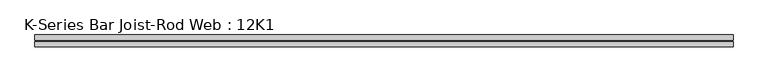
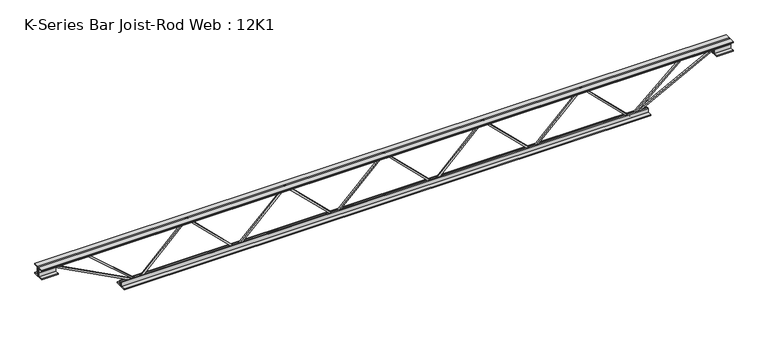
"""IFC4 building model written with IfcOpenShell, lengths in millimetres: beam geometry, K-Series Bar Joist-Rod Web : 12K1."""

from ifc_helpers import new_model, si_unit, frame, origin, place, context, project, spatial, polyline, outline, extrude, source, transform, mapped, element, save


def k_series_bar_joist_rod_web_12k1_62c0aeb9(model_context):
    return source(origin(), model_context, "Body", "SweptSolid", [
        extrude(outline(polyline([(-141.2875, 304.00625), (-150.8125, 304.00625), (-150.8125, 309.1277103), (141.2875, 606.7839603), (141.2875, 609.2410397), (-150.8125, 906.8972897), (-150.8125, 912.01875), (-141.2875, 912.01875), (-141.2875, 910.7902103), (150.8125, 613.1339603), (150.8125, 602.8910397), (-141.2875, 305.2347897), (-141.2875, 304.00625)])), frame((0.0, -4.7625, 0.0), z_axis=(0.0, 1.0, 0.0), x_axis=(0.0, 0.0, 1.0)), (0.0, 0.0, 1.0), 9.525),
        extrude(outline(polyline([(-141.2875, -304.00625), (-150.8125, -304.00625), (-150.8125, -298.8847897), (141.2875, -1.2285397), (141.2875, 1.2285397), (-150.8125, 298.8847897), (-150.8125, 304.00625), (-141.2875, 304.00625), (-141.2875, 302.7777103), (150.8125, 5.1214603), (150.8125, -5.1214603), (-141.2875, -302.7777103), (-141.2875, -304.00625)])), frame((0.0, -4.7625, 0.0), z_axis=(0.0, 1.0, 0.0), x_axis=(0.0, 0.0, 1.0)), (0.0, 0.0, 1.0), 9.525),
        extrude(outline(polyline([(-141.2875, -912.01875), (-150.8125, -912.01875), (-150.8125, -906.8972897), (141.2875, -609.2410397), (141.2875, -606.7839603), (-150.8125, -309.1277103), (-150.8125, -304.00625), (-141.2875, -304.00625), (-141.2875, -305.2347897), (150.8125, -602.8910397), (150.8125, -613.1339603), (-141.2875, -910.7902103), (-141.2875, -912.01875)])), frame((0.0, -4.7625, 0.0), z_axis=(0.0, 1.0, 0.0), x_axis=(0.0, 0.0, 1.0)), (0.0, 0.0, 1.0), 9.525),
        extrude(outline(polyline([(-141.2875, 912.01875), (-150.8125, 912.01875), (-150.8125, 917.1402103), (141.2875, 1214.7964603), (141.2875, 1217.2535397), (-150.8125, 1514.9097897), (-150.8125, 1520.03125), (-141.2875, 1520.03125), (-141.2875, 1518.8027103), (150.8125, 1221.1464603), (150.8125, 1210.9035397), (-141.2875, 913.2472897), (-141.2875, 912.01875)])), frame((0.0, -4.7625, 0.0), z_axis=(0.0, 1.0, 0.0), x_axis=(0.0, 0.0, 1.0)), (0.0, 0.0, 1.0), 9.525),
        extrude(outline(polyline([(-141.2875, -1520.03125), (-150.8125, -1520.03125), (-150.8125, -1514.9097897), (141.2875, -1217.2535397), (141.2875, -1214.7964603), (-150.8125, -917.1402103), (-150.8125, -912.01875), (-141.2875, -912.01875), (-141.2875, -913.2472897), (150.8125, -1210.9035397), (150.8125, -1221.1464603), (-141.2875, -1518.8027103), (-141.2875, -1520.03125)])), frame((0.0, -4.7625, 0.0), z_axis=(0.0, 1.0, 0.0), x_axis=(0.0, 0.0, 1.0)), (0.0, 0.0, 1.0), 9.525),
        extrude(outline(polyline([(4.7625, 152.4), (36.5125, 152.4), (36.5125, 146.05), (11.1125, 146.05), (11.1125, 120.65), (4.7625, 120.65), (4.7625, 152.4)])), frame((-2129.63125, 0.0, 0.0), z_axis=(1.0, 0.0, 0.0), x_axis=(0.0, 1.0, 0.0)), (0.0, 0.0, 1.0), 4259.2625),
        extrude(outline(polyline([(-4.7625, 152.4), (-4.7625, 120.65), (-11.1125, 120.65), (-11.1125, 146.05), (-36.5125, 146.05), (-36.5125, 152.4), (-4.7625, 152.4)])), frame((-2129.63125, 0.0, 0.0), z_axis=(1.0, 0.0, 0.0), x_axis=(0.0, 1.0, 0.0)), (0.0, 0.0, 1.0), 4259.2625),
        extrude(outline(polyline([(-4.7625, 88.9), (-36.5125, 88.9), (-36.5125, 95.25), (-11.1125, 95.25), (-11.1125, 120.65), (-4.7625, 120.65), (-4.7625, 88.9)])), frame((-2129.63125, 0.0, 0.0), z_axis=(1.0, 0.0, 0.0), x_axis=(0.0, 1.0, 0.0)), (0.0, 0.0, 1.0), 101.6),
        extrude(outline(polyline([(36.5125, 88.9), (4.7625, 88.9), (4.7625, 120.65), (11.1125, 120.65), (11.1125, 95.25), (36.5125, 95.25), (36.5125, 88.9)])), frame((-2129.63125, 0.0, 0.0), z_axis=(1.0, 0.0, 0.0), x_axis=(0.0, 1.0, 0.0)), (0.0, 0.0, 1.0), 101.6),
        extrude(outline(polyline([(4.7625, 88.9), (4.7625, 120.65), (11.1125, 120.65), (11.1125, 95.25), (36.5125, 95.25), (36.5125, 88.9), (4.7625, 88.9)])), frame((2028.03125, 0.0, 0.0), z_axis=(1.0, 0.0, 0.0), x_axis=(0.0, 1.0, 0.0)), (0.0, 0.0, 1.0), 101.6),
        extrude(outline(polyline([(-4.7625, 88.9), (-36.5125, 88.9), (-36.5125, 95.25), (-11.1125, 95.25), (-11.1125, 120.65), (-4.7625, 120.65), (-4.7625, 88.9)])), frame((2028.03125, 0.0, 0.0), z_axis=(1.0, 0.0, 0.0), x_axis=(0.0, 1.0, 0.0)), (0.0, 0.0, 1.0), 101.6),
        extrude(outline(polyline([(4.7625, -152.4), (4.7625, -120.65), (11.1125, -120.65), (11.1125, -146.05), (36.5125, -146.05), (36.5125, -152.4), (4.7625, -152.4)])), frame((-1621.63125, 0.0, 0.0), z_axis=(1.0, 0.0, 0.0), x_axis=(0.0, 1.0, 0.0)), (0.0, 0.0, 1.0), 3243.2625),
        extrude(outline(polyline([(-4.7625, -152.4), (-36.5125, -152.4), (-36.5125, -146.05), (-11.1125, -146.05), (-11.1125, -120.65), (-4.7625, -120.65), (-4.7625, -152.4)])), frame((-1621.63125, 0.0, 0.0), z_axis=(1.0, 0.0, 0.0), x_axis=(0.0, 1.0, 0.0)), (0.0, 0.0, 1.0), 3243.2625),
        extrude(outline(polyline([(0.0, -9.525), (0.0, 0.0), (573.7533355, 0.0), (573.7533355, -9.525), (0.0, -9.525)])), frame((-2030.2450214, 4.7625, 116.4332925), z_axis=(0.46483389898951394, 0.0, 0.8853979028381569), x_axis=(0.8853979028381569, 0.0, -0.46483389898951394)), (0.0, 0.0, 1.0), 9.525),
        extrude(outline(polyline([(0.0, -9.525), (0.0, 0.0), (404.4115355, 0.0), (404.4115355, -9.525), (0.0, -9.525)])), frame((-1827.178258, 4.7625, 117.0699098), z_axis=(0.6594767374163246, 0.0, 0.7517249715199835), x_axis=(0.7517249715199835, 0.0, -0.6594767374163246)), (0.0, 0.0, 1.0), 9.525),
        extrude(outline(polyline([(0.0, -9.525), (0.0, 0.0), (573.7533355, 0.0), (573.7533355, -9.525), (0.0, -9.525)])), frame((2030.2450214, -4.7625, 116.4332925), z_axis=(-0.4648338989894953, 0.0, 0.8853979028381667), x_axis=(-0.8853979028381667, 0.0, -0.4648338989894953)), (0.0, 0.0, 1.0), 9.525),
        extrude(outline(polyline([(0.0, -9.525), (0.0, 0.0), (404.4115355, 0.0), (404.4115355, -9.525), (0.0, -9.525)])), frame((1827.178258, -4.7625, 117.0699098), z_axis=(-0.6594767374163193, 0.0, 0.7517249715199882), x_axis=(-0.7517249715199882, 0.0, -0.6594767374163193)), (0.0, 0.0, 1.0), 9.525),
    ])


if __name__ == "__main__":
    model = new_model("IFC4")
    model_context = context("Model", 3, world=origin())
    ifc_project = project(units=[si_unit("LENGTHUNIT", "METRE", prefix="MILLI")], contexts=[model_context])
    site = spatial("IfcSite", under=ifc_project)
    building = spatial("IfcBuilding", under=site)
    placement = place(None, origin())
    k_series_bar_joist_rod_web_12k1_shape = k_series_bar_joist_rod_web_12k1_62c0aeb9(model_context)
    element("IfcBeam", 1, ObjectType="K-Series Bar Joist-Rod Web : 12K1", at=placement, inside=building, context=model_context, shape_type="MappedRepresentation", body=[
        mapped(k_series_bar_joist_rod_web_12k1_shape, transform((0.0, 0.0, 0.0), x_axis=(1.0, 0.0, 0.0), y_axis=(0.0, 1.0, 0.0), z_axis=(0.0, 0.0, 1.0))),
    ])
    save(model, "model.ifc")

# Revit data of these elements
# Type "K-Series Bar Joist-Rod Web : 12K1"
#   Assembly Code = "B1010350"
#   Wt = 5
#   Web Thickness = 0' - 0 3/8"
#   Start Offset [instance default] = 0' - 0"
#   Start Extension [instance default] = 0' - 0"
#   Seat Length = 0' - 4"
#   Seat Depth = 0' - 2 1/2"
#   PanelArrayLength [instance default] = 20' - 0"
#   Panel [instance default] = 2' - 0"
#   End Offset [instance default] = 0' - 0"
#   End Extension [instance default] = 0' - 0"
#   End Panel = 2' - 0"
#   Cord Leg = 0' - 1 1/4"
#   Chord Thickness = 0' - 0 1/4"
#   Length [instance default] = 24' - 0"
#   Depth = 1' - 0"
#   PanelArrayNum [instance default] = 10
#   Structural Material = none
# Element 1 (IfcBeam, "K-Series Bar Joist-Rod Web : 12K1")
#   PanelArrayLength = 9' - 11 11/16"
#   Panel = 1' - 11 15/16"
#   PanelArrayNum = 5
